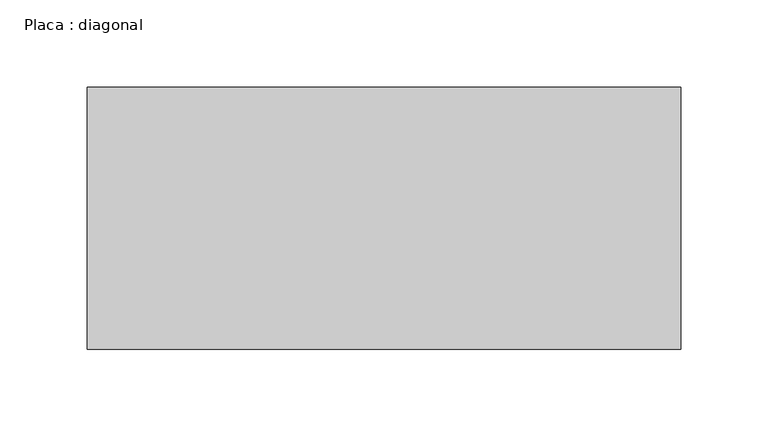
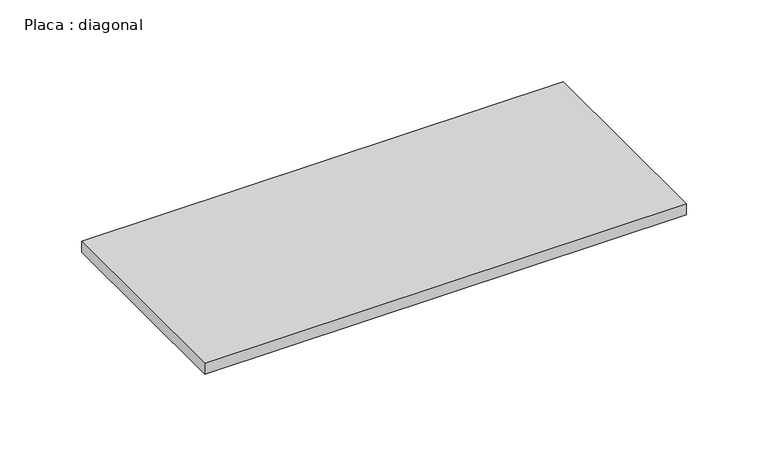
"""IFC4 building model written with IfcOpenShell, lengths in millimetres: beam geometry, Placa : diagonal."""

from ifc_helpers import new_model, si_unit, frame, origin, place, context, project, spatial, polyline, outline, extrude, source, transform, mapped, element, save


def placa_diagonal_fb53ba7d(model_context):
    return source(origin(), model_context, "Body", "SweptSolid", [
        extrude(outline(polyline([(169.971959, 75.0), (169.971959, -75.0), (-169.5739242, -75.0), (-169.5739242, 75.0), (169.971959, 75.0)])), frame((0.0, 0.0, -4.0), z_axis=(0.0, 0.0, 1.0), x_axis=(1.0, 0.0, 0.0)), (0.0, 0.0, 1.0), 8.0),
    ])


if __name__ == "__main__":
    model = new_model("IFC4")
    model_context = context("Model", 3, world=origin())
    ifc_project = project(units=[si_unit("LENGTHUNIT", "METRE", prefix="MILLI")], contexts=[model_context])
    site = spatial("IfcSite", under=ifc_project)
    building = spatial("IfcBuilding", under=site)
    placement = place(None, origin())
    placa_diagonal_shape = placa_diagonal_fb53ba7d(model_context)
    element("IfcBeam", 1, ObjectType="Placa : diagonal", at=placement, inside=building, context=model_context, shape_type="MappedRepresentation", body=[
        mapped(placa_diagonal_shape, transform((0.0, 0.0, 0.0), x_axis=(1.0, 0.0, 0.0), y_axis=(0.0, 1.0, 0.0), z_axis=(0.0, 0.0, 1.0))),
    ])
    save(model, "model.ifc")

# Revit data of these elements
# Type "Placa : diagonal"
#   W = 0
#   Length [instance default] = 1.50 m
#   b = 0.15 m
#   d = 0.008 m
#   A = 0 m²
#   Structural Material [instance default] = Aço, 45-345
# Element 1 (IfcBeam, "Placa : diagonal")
#   Materials on its faces: "Aço, 45-345"
# Materials
#   "Aço, 45-345": class "Metal", colour RGB 247 247 247, transparency 0, Description = "Aço 345 MPa", Cost = 0
